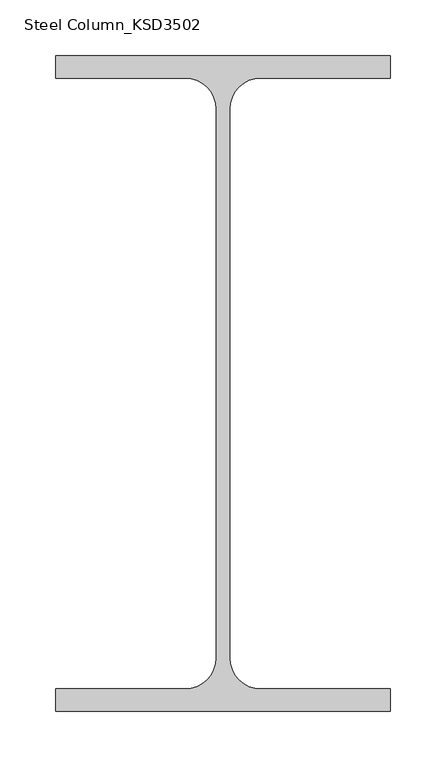
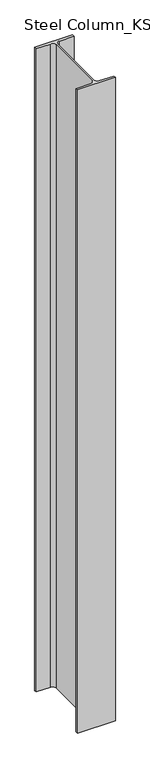
"""IFC4 building model written with IfcOpenShell, lengths in millimetres: column geometry, Steel Column_KSD3502 : H_SC_ASC_H-588×300x12x20."""

import ifcopenshell
import ifcopenshell.guid

model = None  # the IFC model being written
_history = None  # IfcOwnerHistory: only IFC2X3 demands one
_inside = {}  # id of a spatial element -> (the spatial element, [elements in it])
_under = {}  # id of a project, library or spatial element -> (it, [spatial elements below it])
_declared = {}  # id of a project -> (the project, [libraries it declares])
_typed = {}  # id of a type object -> (the type object, [elements of that type])
_made_of = {}  # id of a material, layer set ... -> (it, [elements and type objects made of it])


def new_model(schema):
    """Start an empty IFC model of exactly this schema.

    Asked for "IFC4X3", IfcOpenShell would pick the latest addendum, in which some entities
    have other attributes; the version numbers below select the first issue.
    IFC2X3 requires an IfcOwnerHistory on every rooted entity: one is made here for all.
    """
    global model, _history
    if schema == "IFC4X3":
        model = ifcopenshell.file(schema_version=(4, 3, 0, 0))
    else:
        model = ifcopenshell.file(schema=schema)
    _inside.clear()
    _under.clear()
    _declared.clear()
    _typed.clear()
    _made_of.clear()
    _history = None
    if model.schema == "IFC2X3":
        org = make("IfcOrganization", Name="unknown")
        user = make(
            "IfcPersonAndOrganization",
            ThePerson=make("IfcPerson", FamilyName="unknown"),
            TheOrganization=org,
        )
        app = make(
            "IfcApplication",
            ApplicationDeveloper=org,
            Version="unknown",
            ApplicationFullName="unknown",
            ApplicationIdentifier="unknown",
        )
        _history = make(
            "IfcOwnerHistory",
            OwningUser=user,
            OwningApplication=app,
            ChangeAction="ADDED",
            CreationDate=0,
        )
    return model


def make(cls, **values):
    """One entity of the class cls with the attributes given. An attribute that is None is left unset."""
    return model.create_entity(
        cls, **{name: value for name, value in values.items() if value is not None}
    )


def rooted(cls, **values):
    """An entity with a GlobalId (a new one), such as an element, a storey or a relation."""
    return make(cls, GlobalId=ifcopenshell.guid.new(), OwnerHistory=_history, **values)


def si_unit(unit_type, name, prefix=None):
    """IfcSIUnit, for example si_unit("LENGTHUNIT", "METRE", prefix="MILLI")."""
    return make("IfcSIUnit", UnitType=unit_type, Prefix=prefix, Name=name)


def assignment(units):
    """IfcUnitAssignment: the units of a project."""
    return None if units is None else make("IfcUnitAssignment", Units=units)


def point(xyz):
    """IfcCartesianPoint."""
    return None if xyz is None else make("IfcCartesianPoint", Coordinates=xyz)


def direction(xyz):
    """IfcDirection."""
    return None if xyz is None else make("IfcDirection", DirectionRatios=xyz)


def frame(location, z_axis=None, x_axis=None):
    """IfcAxis2Placement3D, a coordinate frame: its origin and axes. An axis left out is left unset."""
    return make(
        "IfcAxis2Placement3D",
        Location=point(location),
        Axis=direction(z_axis),
        RefDirection=direction(x_axis),
    )


def frame_2d(location, x_axis=None):
    """IfcAxis2Placement2D, a coordinate frame in the plane: its origin and x axis."""
    return make(
        "IfcAxis2Placement2D", Location=point(location), RefDirection=direction(x_axis)
    )


def origin():
    """The frame at (0, 0, 0) with its axes left unset."""
    return frame((0.0, 0.0, 0.0))


def place(relative_to, where):
    """IfcLocalPlacement: puts the frame where relative to a parent placement (None: the world)."""
    return make(
        "IfcLocalPlacement", PlacementRelTo=relative_to, RelativePlacement=where
    )


def context(
    kind, dimensions, precision=None, world=None, true_north=None, identifier=None
):
    """IfcGeometricRepresentationContext, for example the 3D "Model" context."""
    return make(
        "IfcGeometricRepresentationContext",
        ContextIdentifier=identifier,
        ContextType=kind,
        CoordinateSpaceDimension=dimensions,
        Precision=precision,
        WorldCoordinateSystem=world,
        TrueNorth=true_north,
    )


def project(units=None, contexts=None):
    """IfcProject with its units and contexts."""
    return rooted(
        "IfcProject",
        Name="project",
        RepresentationContexts=contexts,
        UnitsInContext=assignment(units),
    )


def spatial(cls, under=None, at=None, **own):
    """A site, building, storey or space (cls), placed at a placement, below another one or the project."""
    s = rooted(cls, ObjectPlacement=at, **own)
    if under is not None:
        _under.setdefault(under.id(), (under, []))[1].append(s)
    return s


def polyline(points):
    """IfcPolyline through the points."""
    return make("IfcPolyline", Points=[point(p) for p in points])


def circle_curve(where, radius):
    """IfcCircle in the frame where."""
    return make("IfcCircle", Position=where, Radius=radius)


def trimmed(basis, trim1, trim2, sense, master):
    """IfcTrimmedCurve: the piece of a basis curve between two trims."""
    return make(
        "IfcTrimmedCurve",
        BasisCurve=basis,
        Trim1=trim1,
        Trim2=trim2,
        SenseAgreement=sense,
        MasterRepresentation=master,
    )


def segment(curve, same_sense, transition):
    """IfcCompositeCurveSegment."""
    return make(
        "IfcCompositeCurveSegment",
        Transition=transition,
        SameSense=same_sense,
        ParentCurve=curve,
    )


def composite_curve(segments, self_intersect=None):
    """IfcCompositeCurve: segments joined end to end."""
    return make("IfcCompositeCurve", Segments=segments, SelfIntersect=self_intersect)


def outline(outer, holes=None, kind="AREA"):
    """IfcArbitraryClosedProfileDef: a profile drawn as a closed curve; with holes, ...WithVoids."""
    if holes is None:
        return make("IfcArbitraryClosedProfileDef", ProfileType=kind, OuterCurve=outer)
    return make(
        "IfcArbitraryProfileDefWithVoids",
        ProfileType=kind,
        OuterCurve=outer,
        InnerCurves=holes,
    )


def extrude(swept, where, along, depth):
    """IfcExtrudedAreaSolid: the profile swept, set in the frame where, extruded along a direction by depth."""
    return make(
        "IfcExtrudedAreaSolid",
        SweptArea=swept,
        Position=where,
        ExtrudedDirection=direction(along),
        Depth=depth,
    )


def shape(context_of_items, identifier, shape_type, items):
    """IfcShapeRepresentation: the items that make up one representation, for example the "Body"."""
    return make(
        "IfcShapeRepresentation",
        ContextOfItems=context_of_items,
        RepresentationIdentifier=identifier,
        RepresentationType=shape_type,
        Items=items,
    )


def source(mapping_origin, context_of_items, identifier, shape_type, items):
    """IfcRepresentationMap: a shape defined once, which mapped items show again and again."""
    return make(
        "IfcRepresentationMap",
        MappingOrigin=mapping_origin,
        MappedRepresentation=shape(context_of_items, identifier, shape_type, items),
    )


def transform(
    local_origin,
    x_axis=None,
    y_axis=None,
    z_axis=None,
    scale=None,
    scale2=None,
    scale3=None,
    uniform=True,
):
    """IfcCartesianTransformationOperator3D, or its non-uniform kind. x_axis, y_axis, z_axis: its Axis1, 2, 3."""
    if uniform:
        return make(
            "IfcCartesianTransformationOperator3D",
            Axis1=direction(x_axis),
            Axis2=direction(y_axis),
            LocalOrigin=point(local_origin),
            Scale=scale,
            Axis3=direction(z_axis),
        )
    return make(
        "IfcCartesianTransformationOperator3DnonUniform",
        Axis1=direction(x_axis),
        Axis2=direction(y_axis),
        LocalOrigin=point(local_origin),
        Scale=scale,
        Axis3=direction(z_axis),
        Scale2=scale2,
        Scale3=scale3,
    )


def mapped(mapping_source, mapping_target):
    """IfcMappedItem: shows the shape of a source again, moved by a transform."""
    return make(
        "IfcMappedItem", MappingSource=mapping_source, MappingTarget=mapping_target
    )


def made_of(thing, what):
    """Note that an element or type object is made of a material, layer set ...; save() writes the relation."""
    if what is not None:
        _made_of.setdefault(what.id(), (what, []))[1].append(thing)
    return thing


def element(
    cls,
    number,
    at=None,
    inside=None,
    cuts=None,
    type_object=None,
    material=None,
    context=None,
    identifier="Body",
    shape_type=None,
    held_by="IfcProductDefinitionShape",
    body=None,
    shapes=None,
    **own,
):
    """One element of the class cls, such as IfcWall. Its Tag is "e" and its number.

    at: its placement. inside: the storey or other place that contains it. cuts: it is an
    opening in that element (IfcRelVoidsElement). A single representation is given by context,
    identifier, shape_type and body (its items); several are given by shapes. held_by: the class
    of the entity that holds the representations. save() writes the other relations.
    """
    e = rooted(cls, Tag="e%d" % number, ObjectPlacement=at, **own)
    if body is not None:
        shapes = [shape(context, identifier, shape_type, body)]
    if shapes is not None:
        e.Representation = make(held_by, Representations=shapes)
    if inside is not None:
        _inside.setdefault(inside.id(), (inside, []))[1].append(e)
    if cuts is not None:
        rooted(
            "IfcRelVoidsElement", RelatingBuildingElement=cuts, RelatedOpeningElement=e
        )
    if type_object is not None:
        _typed.setdefault(type_object.id(), (type_object, []))[1].append(e)
    return made_of(e, material)


def aggregate(whole, parts):
    """IfcRelAggregates: a whole, such as a stair, and the parts it consists of."""
    return rooted("IfcRelAggregates", RelatingObject=whole, RelatedObjects=parts)


def save(model, path):
    """Write the relations noted so far, then the file.

    IfcRelAggregates (storeys below a building ...), IfcRelContainedInSpatialStructure (elements
    in a storey), IfcRelDefinesByType, IfcRelAssociatesMaterial and IfcRelDeclares: one each for
    every whole, place, type object, material and project.
    """
    for whole, parts in _under.values():
        aggregate(whole, parts)
    for where, things in _inside.values():
        rooted(
            "IfcRelContainedInSpatialStructure",
            RelatedElements=things,
            RelatingStructure=where,
        )
    for kind, things in _typed.values():
        rooted("IfcRelDefinesByType", RelatedObjects=things, RelatingType=kind)
    for what, things in _made_of.values():
        rooted("IfcRelAssociatesMaterial", RelatedObjects=things, RelatingMaterial=what)
    for by, libraries in _declared.values():
        rooted("IfcRelDeclares", RelatingContext=by, RelatedDefinitions=libraries)
    model.write(path)


def steel_column_ksd3502_190025ee(model_context):
    return source(origin(), model_context, "Body", "SweptSolid", [
        extrude(outline(composite_curve([segment(polyline([(150.0, 294.0), (150.0, 274.0), (34.0, 274.0)]), True, "CONTINUOUS"), segment(trimmed(circle_curve(frame_2d((34.0, 246.0)), 28.0), [point((34.0, 274.0))], [point((6.0, 246.0))], True, "CARTESIAN"), True, "CONTINUOUS"), segment(polyline([(6.0, 246.0), (6.0, -246.0)]), True, "CONTINUOUS"), segment(trimmed(circle_curve(frame_2d((34.0, -246.0)), 28.0), [point((6.0, -246.0))], [point((34.0, -274.0))], True, "CARTESIAN"), True, "CONTINUOUS"), segment(polyline([(34.0, -274.0), (150.0, -274.0), (150.0, -294.0), (-150.0, -294.0), (-150.0, -274.0), (-34.0, -274.0)]), True, "CONTINUOUS"), segment(trimmed(circle_curve(frame_2d((-34.0, -246.0)), 28.0), [point((-34.0, -274.0))], [point((-6.0, -246.0))], True, "CARTESIAN"), True, "CONTINUOUS"), segment(polyline([(-6.0, -246.0), (-6.0, 246.0)]), True, "CONTINUOUS"), segment(trimmed(circle_curve(frame_2d((-34.0, 246.0)), 28.0), [point((-6.0, 246.0))], [point((-34.0, 274.0))], True, "CARTESIAN"), True, "CONTINUOUS"), segment(polyline([(-34.0, 274.0), (-150.0, 274.0), (-150.0, 294.0), (150.0, 294.0)]), True, "CONTINUOUS")], self_intersect=False)), frame((0.0, 0.0, 11909.9720055), z_axis=(0.0, 0.0, 1.0), x_axis=(1.0, 0.0, 0.0)), (0.0, 0.0, 1.0), 5390.0),
    ])


if __name__ == "__main__":
    model = new_model("IFC4")
    model_context = context("Model", 3, world=origin())
    ifc_project = project(units=[si_unit("LENGTHUNIT", "METRE", prefix="MILLI")], contexts=[model_context])
    site = spatial("IfcSite", under=ifc_project)
    building = spatial("IfcBuilding", under=site)
    placement = place(None, origin())
    steel_column_ksd3502_shape = steel_column_ksd3502_190025ee(model_context)
    element("IfcColumn", 1, ObjectType="Steel Column_KSD3502 : H_SC_ASC_H-588×300x12x20", at=placement, inside=building, context=model_context, shape_type="MappedRepresentation", body=[
        mapped(steel_column_ksd3502_shape, transform((0.0, 0.0, 0.0), x_axis=(1.0, 0.0, 0.0), y_axis=(0.0, 1.0, 0.0), z_axis=(0.0, 0.0, 1.0))),
    ])
    save(model, "model.ifc")

# Revit data of these elements
# Type "Steel Column_KSD3502 : H_SC_ASC_H-588×300x12x20"
#   Width = 30.0 cm
#   Web Thickness = 1.2 cm
#   Web Fillet = 2.8 cm
#   Warping Constant = 7259040.0 cm⁶
#   Torsional Moment of Inertia = 192.717 cm⁴
#   Section Area = 192.5 cm²
#   Plastic Modulus weak axis = 928.0 cm³
#   Plastic Modulus strong axis = 4490.0 cm³
#   Perimeter = 1.27 m²/m
#   Nominal Weight = 151.00 kgf/m
#   Moment of Inertia weak axis = 9020.00 cm⁴
#   Moment of Inertia strong axis = 118000.00 cm⁴
#   Height = 58.8 cm
#   Flange Thickness = 2.0 cm
#   Elastic Modulus weak axis = 601.0 cm³
#   Elastic Modulus strong axis = 4020.0 cm³
#   Centroid Vertical = 29.4 cm
#   Centroid Horizontal = 15.0 cm
#   Bolt Spacing = 13.97 cm
#   Structural Material [instance default] = Steel, 45-345
#   Section Name Key = ""
#   Assembly Code = ""
# Element 1 (IfcColumn, "Steel Column_KSD3502 : H_SC_ASC_H-588×300x12x20")
#   Structural Material = none
# Materials
#   "Steel, 45-345": class "Metal", colour RGB 189 187 185, transparency 0, Description = "Steel 345 MPa", Cost = 0
